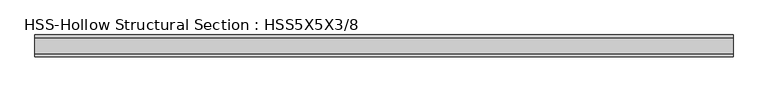
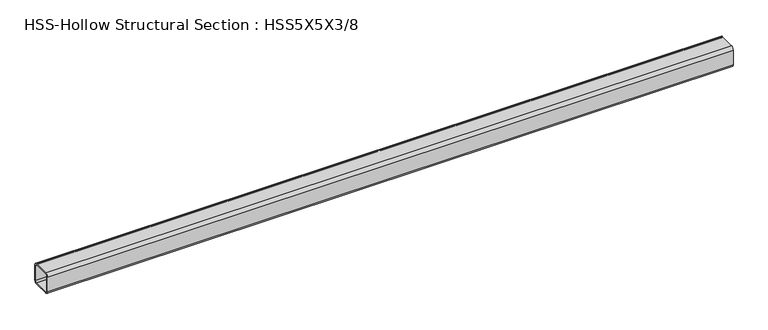
"""IFC4 building model written with IfcOpenShell, lengths in millimetres: member geometry, HSS-Hollow Structural Section : HSS5X5X3/8."""

import ifcopenshell
import ifcopenshell.guid

model = None  # the IFC model being written
_history = None  # IfcOwnerHistory: only IFC2X3 demands one
_inside = {}  # id of a spatial element -> (the spatial element, [elements in it])
_under = {}  # id of a project, library or spatial element -> (it, [spatial elements below it])
_declared = {}  # id of a project -> (the project, [libraries it declares])
_typed = {}  # id of a type object -> (the type object, [elements of that type])
_made_of = {}  # id of a material, layer set ... -> (it, [elements and type objects made of it])


def new_model(schema):
    """Start an empty IFC model of exactly this schema.

    Asked for "IFC4X3", IfcOpenShell would pick the latest addendum, in which some entities
    have other attributes; the version numbers below select the first issue.
    IFC2X3 requires an IfcOwnerHistory on every rooted entity: one is made here for all.
    """
    global model, _history
    if schema == "IFC4X3":
        model = ifcopenshell.file(schema_version=(4, 3, 0, 0))
    else:
        model = ifcopenshell.file(schema=schema)
    _inside.clear()
    _under.clear()
    _declared.clear()
    _typed.clear()
    _made_of.clear()
    _history = None
    if model.schema == "IFC2X3":
        org = make("IfcOrganization", Name="unknown")
        user = make(
            "IfcPersonAndOrganization",
            ThePerson=make("IfcPerson", FamilyName="unknown"),
            TheOrganization=org,
        )
        app = make(
            "IfcApplication",
            ApplicationDeveloper=org,
            Version="unknown",
            ApplicationFullName="unknown",
            ApplicationIdentifier="unknown",
        )
        _history = make(
            "IfcOwnerHistory",
            OwningUser=user,
            OwningApplication=app,
            ChangeAction="ADDED",
            CreationDate=0,
        )
    return model


def make(cls, **values):
    """One entity of the class cls with the attributes given. An attribute that is None is left unset."""
    return model.create_entity(
        cls, **{name: value for name, value in values.items() if value is not None}
    )


def rooted(cls, **values):
    """An entity with a GlobalId (a new one), such as an element, a storey or a relation."""
    return make(cls, GlobalId=ifcopenshell.guid.new(), OwnerHistory=_history, **values)


def si_unit(unit_type, name, prefix=None):
    """IfcSIUnit, for example si_unit("LENGTHUNIT", "METRE", prefix="MILLI")."""
    return make("IfcSIUnit", UnitType=unit_type, Prefix=prefix, Name=name)


def assignment(units):
    """IfcUnitAssignment: the units of a project."""
    return None if units is None else make("IfcUnitAssignment", Units=units)


def point(xyz):
    """IfcCartesianPoint."""
    return None if xyz is None else make("IfcCartesianPoint", Coordinates=xyz)


def direction(xyz):
    """IfcDirection."""
    return None if xyz is None else make("IfcDirection", DirectionRatios=xyz)


def frame(location, z_axis=None, x_axis=None):
    """IfcAxis2Placement3D, a coordinate frame: its origin and axes. An axis left out is left unset."""
    return make(
        "IfcAxis2Placement3D",
        Location=point(location),
        Axis=direction(z_axis),
        RefDirection=direction(x_axis),
    )


def frame_2d(location, x_axis=None):
    """IfcAxis2Placement2D, a coordinate frame in the plane: its origin and x axis."""
    return make(
        "IfcAxis2Placement2D", Location=point(location), RefDirection=direction(x_axis)
    )


def origin():
    """The frame at (0, 0, 0) with its axes left unset."""
    return frame((0.0, 0.0, 0.0))


def place(relative_to, where):
    """IfcLocalPlacement: puts the frame where relative to a parent placement (None: the world)."""
    return make(
        "IfcLocalPlacement", PlacementRelTo=relative_to, RelativePlacement=where
    )


def context(
    kind, dimensions, precision=None, world=None, true_north=None, identifier=None
):
    """IfcGeometricRepresentationContext, for example the 3D "Model" context."""
    return make(
        "IfcGeometricRepresentationContext",
        ContextIdentifier=identifier,
        ContextType=kind,
        CoordinateSpaceDimension=dimensions,
        Precision=precision,
        WorldCoordinateSystem=world,
        TrueNorth=true_north,
    )


def project(units=None, contexts=None):
    """IfcProject with its units and contexts."""
    return rooted(
        "IfcProject",
        Name="project",
        RepresentationContexts=contexts,
        UnitsInContext=assignment(units),
    )


def spatial(cls, under=None, at=None, **own):
    """A site, building, storey or space (cls), placed at a placement, below another one or the project."""
    s = rooted(cls, ObjectPlacement=at, **own)
    if under is not None:
        _under.setdefault(under.id(), (under, []))[1].append(s)
    return s


def polyline(points):
    """IfcPolyline through the points."""
    return make("IfcPolyline", Points=[point(p) for p in points])


def circle_curve(where, radius):
    """IfcCircle in the frame where."""
    return make("IfcCircle", Position=where, Radius=radius)


def trimmed(basis, trim1, trim2, sense, master):
    """IfcTrimmedCurve: the piece of a basis curve between two trims."""
    return make(
        "IfcTrimmedCurve",
        BasisCurve=basis,
        Trim1=trim1,
        Trim2=trim2,
        SenseAgreement=sense,
        MasterRepresentation=master,
    )


def segment(curve, same_sense, transition):
    """IfcCompositeCurveSegment."""
    return make(
        "IfcCompositeCurveSegment",
        Transition=transition,
        SameSense=same_sense,
        ParentCurve=curve,
    )


def composite_curve(segments, self_intersect=None):
    """IfcCompositeCurve: segments joined end to end."""
    return make("IfcCompositeCurve", Segments=segments, SelfIntersect=self_intersect)


def outline(outer, holes=None, kind="AREA"):
    """IfcArbitraryClosedProfileDef: a profile drawn as a closed curve; with holes, ...WithVoids."""
    if holes is None:
        return make("IfcArbitraryClosedProfileDef", ProfileType=kind, OuterCurve=outer)
    return make(
        "IfcArbitraryProfileDefWithVoids",
        ProfileType=kind,
        OuterCurve=outer,
        InnerCurves=holes,
    )


def extrude(swept, where, along, depth):
    """IfcExtrudedAreaSolid: the profile swept, set in the frame where, extruded along a direction by depth."""
    return make(
        "IfcExtrudedAreaSolid",
        SweptArea=swept,
        Position=where,
        ExtrudedDirection=direction(along),
        Depth=depth,
    )


def shape(context_of_items, identifier, shape_type, items):
    """IfcShapeRepresentation: the items that make up one representation, for example the "Body"."""
    return make(
        "IfcShapeRepresentation",
        ContextOfItems=context_of_items,
        RepresentationIdentifier=identifier,
        RepresentationType=shape_type,
        Items=items,
    )


def source(mapping_origin, context_of_items, identifier, shape_type, items):
    """IfcRepresentationMap: a shape defined once, which mapped items show again and again."""
    return make(
        "IfcRepresentationMap",
        MappingOrigin=mapping_origin,
        MappedRepresentation=shape(context_of_items, identifier, shape_type, items),
    )


def transform(
    local_origin,
    x_axis=None,
    y_axis=None,
    z_axis=None,
    scale=None,
    scale2=None,
    scale3=None,
    uniform=True,
):
    """IfcCartesianTransformationOperator3D, or its non-uniform kind. x_axis, y_axis, z_axis: its Axis1, 2, 3."""
    if uniform:
        return make(
            "IfcCartesianTransformationOperator3D",
            Axis1=direction(x_axis),
            Axis2=direction(y_axis),
            LocalOrigin=point(local_origin),
            Scale=scale,
            Axis3=direction(z_axis),
        )
    return make(
        "IfcCartesianTransformationOperator3DnonUniform",
        Axis1=direction(x_axis),
        Axis2=direction(y_axis),
        LocalOrigin=point(local_origin),
        Scale=scale,
        Axis3=direction(z_axis),
        Scale2=scale2,
        Scale3=scale3,
    )


def mapped(mapping_source, mapping_target):
    """IfcMappedItem: shows the shape of a source again, moved by a transform."""
    return make(
        "IfcMappedItem", MappingSource=mapping_source, MappingTarget=mapping_target
    )


def made_of(thing, what):
    """Note that an element or type object is made of a material, layer set ...; save() writes the relation."""
    if what is not None:
        _made_of.setdefault(what.id(), (what, []))[1].append(thing)
    return thing


def element(
    cls,
    number,
    at=None,
    inside=None,
    cuts=None,
    type_object=None,
    material=None,
    context=None,
    identifier="Body",
    shape_type=None,
    held_by="IfcProductDefinitionShape",
    body=None,
    shapes=None,
    **own,
):
    """One element of the class cls, such as IfcWall. Its Tag is "e" and its number.

    at: its placement. inside: the storey or other place that contains it. cuts: it is an
    opening in that element (IfcRelVoidsElement). A single representation is given by context,
    identifier, shape_type and body (its items); several are given by shapes. held_by: the class
    of the entity that holds the representations. save() writes the other relations.
    """
    e = rooted(cls, Tag="e%d" % number, ObjectPlacement=at, **own)
    if body is not None:
        shapes = [shape(context, identifier, shape_type, body)]
    if shapes is not None:
        e.Representation = make(held_by, Representations=shapes)
    if inside is not None:
        _inside.setdefault(inside.id(), (inside, []))[1].append(e)
    if cuts is not None:
        rooted(
            "IfcRelVoidsElement", RelatingBuildingElement=cuts, RelatedOpeningElement=e
        )
    if type_object is not None:
        _typed.setdefault(type_object.id(), (type_object, []))[1].append(e)
    return made_of(e, material)


def aggregate(whole, parts):
    """IfcRelAggregates: a whole, such as a stair, and the parts it consists of."""
    return rooted("IfcRelAggregates", RelatingObject=whole, RelatedObjects=parts)


def save(model, path):
    """Write the relations noted so far, then the file.

    IfcRelAggregates (storeys below a building ...), IfcRelContainedInSpatialStructure (elements
    in a storey), IfcRelDefinesByType, IfcRelAssociatesMaterial and IfcRelDeclares: one each for
    every whole, place, type object, material and project.
    """
    for whole, parts in _under.values():
        aggregate(whole, parts)
    for where, things in _inside.values():
        rooted(
            "IfcRelContainedInSpatialStructure",
            RelatedElements=things,
            RelatingStructure=where,
        )
    for kind, things in _typed.values():
        rooted("IfcRelDefinesByType", RelatedObjects=things, RelatingType=kind)
    for what, things in _made_of.values():
        rooted("IfcRelAssociatesMaterial", RelatedObjects=things, RelatingMaterial=what)
    for by, libraries in _declared.values():
        rooted("IfcRelDeclares", RelatingContext=by, RelatedDefinitions=libraries)
    model.write(path)


def hss_hollow_structural_section_hss5x5x3_8_d39f42fe(model_context):
    return source(origin(), model_context, "Body", "SweptSolid", [
        extrude(outline(composite_curve([segment(polyline([(63.5, 45.7708), (63.5, -45.7708)]), True, "CONTINUOUS"), segment(trimmed(circle_curve(frame_2d((45.7708, -45.7708)), 17.7292), [point((63.5, -45.7708))], [point((45.7708, -63.5))], False, "CARTESIAN"), True, "CONTINUOUS"), segment(polyline([(45.7708, -63.5), (-45.7708, -63.5)]), True, "CONTINUOUS"), segment(trimmed(circle_curve(frame_2d((-45.7708, -45.7708)), 17.7292), [point((-45.7708, -63.5))], [point((-63.5, -45.7708))], False, "CARTESIAN"), True, "CONTINUOUS"), segment(polyline([(-63.5, -45.7708), (-63.5, 45.7708)]), True, "CONTINUOUS"), segment(trimmed(circle_curve(frame_2d((-45.7708, 45.7708)), 17.7292), [point((-63.5, 45.7708))], [point((-45.7708, 63.5))], False, "CARTESIAN"), True, "CONTINUOUS"), segment(polyline([(-45.7708, 63.5), (45.7708, 63.5)]), True, "CONTINUOUS"), segment(trimmed(circle_curve(frame_2d((45.7708, 45.7708)), 17.7292), [point((45.7708, 63.5))], [point((63.5, 45.7708))], False, "CARTESIAN"), True, "CONTINUOUS")], self_intersect=False), holes=[composite_curve([segment(trimmed(circle_curve(frame_2d((-45.7708, 45.7708)), 8.8646), [point((-45.7708, 54.6354))], [point((-54.6354, 45.7708))], True, "CARTESIAN"), True, "CONTINUOUS"), segment(polyline([(-54.6354, 45.7708), (-54.6354, -45.7708)]), True, "CONTINUOUS"), segment(trimmed(circle_curve(frame_2d((-45.7708, -45.7708)), 8.8646), [point((-54.6354, -45.7708))], [point((-45.7708, -54.6354))], True, "CARTESIAN"), True, "CONTINUOUS"), segment(polyline([(-45.7708, -54.6354), (45.7708, -54.6354)]), True, "CONTINUOUS"), segment(trimmed(circle_curve(frame_2d((45.7708, -45.7708)), 8.8646), [point((45.7708, -54.6354))], [point((54.6354, -45.7708))], True, "CARTESIAN"), True, "CONTINUOUS"), segment(polyline([(54.6354, -45.7708), (54.6354, 45.7708)]), True, "CONTINUOUS"), segment(trimmed(circle_curve(frame_2d((45.7708, 45.7708)), 8.8646), [point((54.6354, 45.7708))], [point((45.7708, 54.6354))], True, "CARTESIAN"), True, "CONTINUOUS"), segment(polyline([(45.7708, 54.6354), (-45.7708, 54.6354)]), True, "CONTINUOUS")], self_intersect=False)]), frame((-2022.2115003, 0.0, 0.0), z_axis=(1.0, 0.0, 0.0), x_axis=(0.0, 1.0, 0.0)), (0.0, 0.0, 1.0), 4044.4230006),
    ])


if __name__ == "__main__":
    model = new_model("IFC4")
    model_context = context("Model", 3, world=origin())
    ifc_project = project(units=[si_unit("LENGTHUNIT", "METRE", prefix="MILLI")], contexts=[model_context])
    site = spatial("IfcSite", under=ifc_project)
    building = spatial("IfcBuilding", under=site)
    placement = place(None, origin())
    hss_hollow_structural_section_hss5x5x3_8_shape = hss_hollow_structural_section_hss5x5x3_8_d39f42fe(model_context)
    element("IfcMember", 1, ObjectType="HSS-Hollow Structural Section : HSS5X5X3/8", at=placement, inside=building, context=model_context, shape_type="MappedRepresentation", body=[
        mapped(hss_hollow_structural_section_hss5x5x3_8_shape, transform((0.0, 0.0, 0.0), x_axis=(1.0, 0.0, 0.0), y_axis=(0.0, 1.0, 0.0), z_axis=(0.0, 0.0, 1.0))),
    ])
    save(model, "model.ifc")

# Revit data of these elements
# Type "HSS-Hollow Structural Section : HSS5X5X3/8"
#   Assembly Code = "B10"
#   Shape = "Square"
#   W = 22.3
#   Ht = 0' - 5"
#   Length [instance default] = 5' - 0"
#   b = 0' - 5"
#   kr = 0' - 0.698"
#   t = 0' - 0.349"
#   A = 0.0429167 SF
#   Structural Material [instance default] = Steel ASTM A500, Grade B, Rectangular and Square
# Element 1 (IfcMember, "HSS-Hollow Structural Section : HSS5X5X3/8")
#   Materials on its faces: "Steel ASTM A500, Grade B, Rectangular and Square"
# Materials
#   "Steel ASTM A500, Grade B, Rectangular and Square": class "Metal", colour RGB 199 199 199, transparency 0, Description = "Carbon steel", Cost = 0
